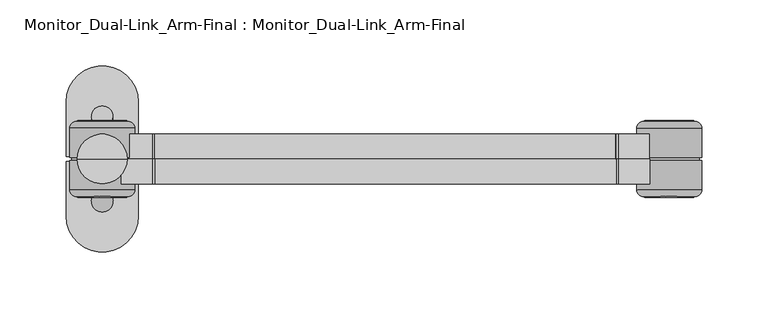
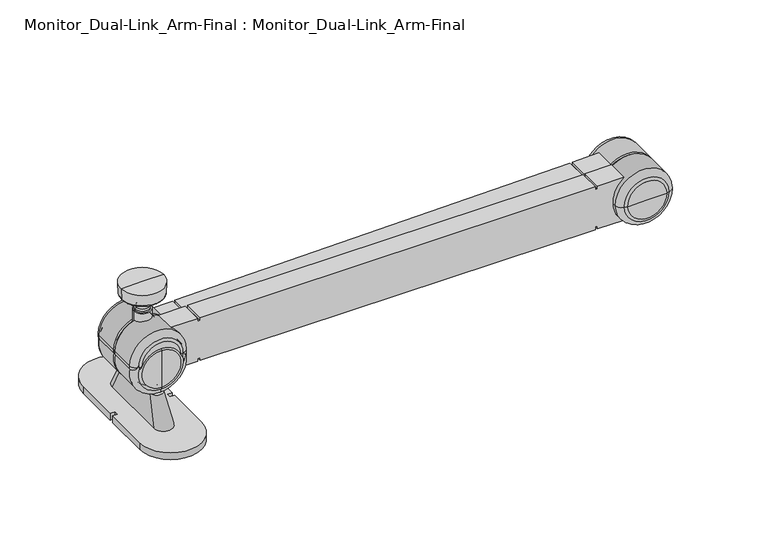
# IFC4 building model written with IfcOpenShell, lengths in millimetres: proxy geometry, Monitor_Dual-Link_Arm-Final : Monitor_Dual-Link_Arm-Final.
# Revit data of these elements (continued)
# Project information
#   Room Abbreviation = "VEX01"
#   Room Description = "Exam/Treatment, Veterinary (VEX01)"
#   Sheets - Total = "5"
#   Project Issue Date = "Issue Date"
#   Project Status = "Project Status"
#   Client Name = "Owner"
#   Project Address = "Enter address here"
#   Project Name = "Project Name"
#   Project Number = "Project Number"
#   Publication Date = "30-Jan-15"
# Type "Monitor_Dual-Link_Arm-Final : Monitor_Dual-Link_Arm-Final"
#   Real Monitor Angle [instance default] = 90.00°
#   Real MAngle Arm2 [instance default] = 90.00°
#   Real MAngle Arm1 [instance default] = 90.00°
#   Length M2 [instance default] = 1' - 4 7/8"
#   Length M1 [instance default] = 1' - 4 7/8"
#   Monitor Base Angle [instance default] = 90.00°
#   MArm Angle2 [instance default] = 90.00°
#   MArm Angle1 [instance default] = 90.00°
#   Screen Texture = none
#   MArms Texture [instance default] = none
#   Default Elevation = 0
# Element 1 (IfcBuildingElementProxy, "Monitor_Dual-Link_Arm-Final : Monitor_Dual-Link_Arm-Final")
#   Real MAngle Arm2 = 180.00°
#   Real MAngle Arm1 = 1.00°
#   MArm Angle2 = 180.00°
#   MArm Angle1 = 0.00°
#   MArms Texture = Arm_Other Texture
#   Materials on its faces: "Arm_Other Texture"
# Materials
#   "Arm_Other Texture": class "Unassigned", colour RGB 196 193 204, transparency 0
